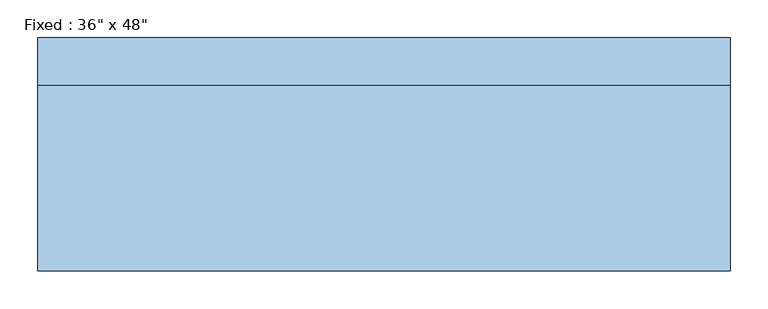
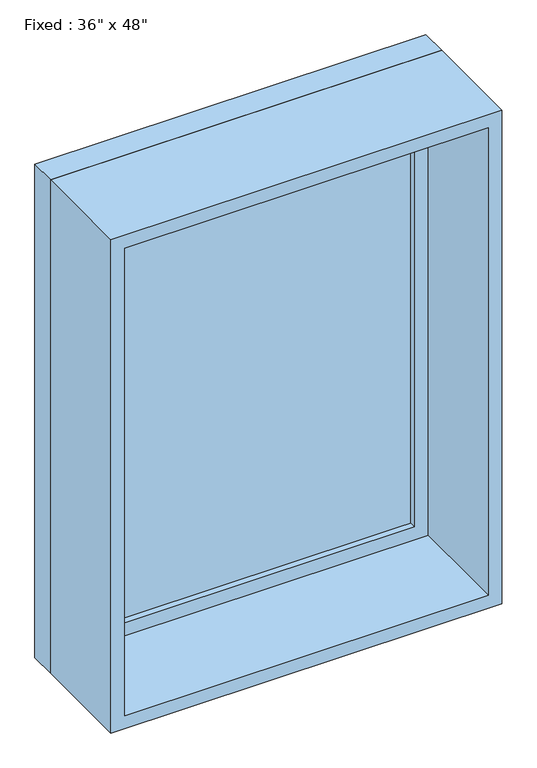
"""IFC4 building model written with IfcOpenShell, lengths in millimetres: window geometry."""

import ifcopenshell
import ifcopenshell.guid

model = None  # the IFC model being written
_history = None  # IfcOwnerHistory: only IFC2X3 demands one
_inside = {}  # id of a spatial element -> (the spatial element, [elements in it])
_under = {}  # id of a project, library or spatial element -> (it, [spatial elements below it])
_declared = {}  # id of a project -> (the project, [libraries it declares])
_typed = {}  # id of a type object -> (the type object, [elements of that type])
_made_of = {}  # id of a material, layer set ... -> (it, [elements and type objects made of it])


def new_model(schema):
    """Start an empty IFC model of exactly this schema.

    Asked for "IFC4X3", IfcOpenShell would pick the latest addendum, in which some entities
    have other attributes; the version numbers below select the first issue.
    IFC2X3 requires an IfcOwnerHistory on every rooted entity: one is made here for all.
    """
    global model, _history
    if schema == "IFC4X3":
        model = ifcopenshell.file(schema_version=(4, 3, 0, 0))
    else:
        model = ifcopenshell.file(schema=schema)
    _inside.clear()
    _under.clear()
    _declared.clear()
    _typed.clear()
    _made_of.clear()
    _history = None
    if model.schema == "IFC2X3":
        org = make("IfcOrganization", Name="unknown")
        user = make(
            "IfcPersonAndOrganization",
            ThePerson=make("IfcPerson", FamilyName="unknown"),
            TheOrganization=org,
        )
        app = make(
            "IfcApplication",
            ApplicationDeveloper=org,
            Version="unknown",
            ApplicationFullName="unknown",
            ApplicationIdentifier="unknown",
        )
        _history = make(
            "IfcOwnerHistory",
            OwningUser=user,
            OwningApplication=app,
            ChangeAction="ADDED",
            CreationDate=0,
        )
    return model


def make(cls, **values):
    """One entity of the class cls with the attributes given. An attribute that is None is left unset."""
    return model.create_entity(
        cls, **{name: value for name, value in values.items() if value is not None}
    )


def rooted(cls, **values):
    """An entity with a GlobalId (a new one), such as an element, a storey or a relation."""
    return make(cls, GlobalId=ifcopenshell.guid.new(), OwnerHistory=_history, **values)


def si_unit(unit_type, name, prefix=None):
    """IfcSIUnit, for example si_unit("LENGTHUNIT", "METRE", prefix="MILLI")."""
    return make("IfcSIUnit", UnitType=unit_type, Prefix=prefix, Name=name)


def assignment(units):
    """IfcUnitAssignment: the units of a project."""
    return None if units is None else make("IfcUnitAssignment", Units=units)


def point(xyz):
    """IfcCartesianPoint."""
    return None if xyz is None else make("IfcCartesianPoint", Coordinates=xyz)


def direction(xyz):
    """IfcDirection."""
    return None if xyz is None else make("IfcDirection", DirectionRatios=xyz)


def frame(location, z_axis=None, x_axis=None):
    """IfcAxis2Placement3D, a coordinate frame: its origin and axes. An axis left out is left unset."""
    return make(
        "IfcAxis2Placement3D",
        Location=point(location),
        Axis=direction(z_axis),
        RefDirection=direction(x_axis),
    )


def origin():
    """The frame at (0, 0, 0) with its axes left unset."""
    return frame((0.0, 0.0, 0.0))


def place(relative_to, where):
    """IfcLocalPlacement: puts the frame where relative to a parent placement (None: the world)."""
    return make(
        "IfcLocalPlacement", PlacementRelTo=relative_to, RelativePlacement=where
    )


def context(
    kind, dimensions, precision=None, world=None, true_north=None, identifier=None
):
    """IfcGeometricRepresentationContext, for example the 3D "Model" context."""
    return make(
        "IfcGeometricRepresentationContext",
        ContextIdentifier=identifier,
        ContextType=kind,
        CoordinateSpaceDimension=dimensions,
        Precision=precision,
        WorldCoordinateSystem=world,
        TrueNorth=true_north,
    )


def project(units=None, contexts=None):
    """IfcProject with its units and contexts."""
    return rooted(
        "IfcProject",
        Name="project",
        RepresentationContexts=contexts,
        UnitsInContext=assignment(units),
    )


def spatial(cls, under=None, at=None, **own):
    """A site, building, storey or space (cls), placed at a placement, below another one or the project."""
    s = rooted(cls, ObjectPlacement=at, **own)
    if under is not None:
        _under.setdefault(under.id(), (under, []))[1].append(s)
    return s


def polyline(points):
    """IfcPolyline through the points."""
    return make("IfcPolyline", Points=[point(p) for p in points])


def outline(outer, holes=None, kind="AREA"):
    """IfcArbitraryClosedProfileDef: a profile drawn as a closed curve; with holes, ...WithVoids."""
    if holes is None:
        return make("IfcArbitraryClosedProfileDef", ProfileType=kind, OuterCurve=outer)
    return make(
        "IfcArbitraryProfileDefWithVoids",
        ProfileType=kind,
        OuterCurve=outer,
        InnerCurves=holes,
    )


def extrude(swept, where, along, depth):
    """IfcExtrudedAreaSolid: the profile swept, set in the frame where, extruded along a direction by depth."""
    return make(
        "IfcExtrudedAreaSolid",
        SweptArea=swept,
        Position=where,
        ExtrudedDirection=direction(along),
        Depth=depth,
    )


def shape(context_of_items, identifier, shape_type, items):
    """IfcShapeRepresentation: the items that make up one representation, for example the "Body"."""
    return make(
        "IfcShapeRepresentation",
        ContextOfItems=context_of_items,
        RepresentationIdentifier=identifier,
        RepresentationType=shape_type,
        Items=items,
    )


def source(mapping_origin, context_of_items, identifier, shape_type, items):
    """IfcRepresentationMap: a shape defined once, which mapped items show again and again."""
    return make(
        "IfcRepresentationMap",
        MappingOrigin=mapping_origin,
        MappedRepresentation=shape(context_of_items, identifier, shape_type, items),
    )


def transform(
    local_origin,
    x_axis=None,
    y_axis=None,
    z_axis=None,
    scale=None,
    scale2=None,
    scale3=None,
    uniform=True,
):
    """IfcCartesianTransformationOperator3D, or its non-uniform kind. x_axis, y_axis, z_axis: its Axis1, 2, 3."""
    if uniform:
        return make(
            "IfcCartesianTransformationOperator3D",
            Axis1=direction(x_axis),
            Axis2=direction(y_axis),
            LocalOrigin=point(local_origin),
            Scale=scale,
            Axis3=direction(z_axis),
        )
    return make(
        "IfcCartesianTransformationOperator3DnonUniform",
        Axis1=direction(x_axis),
        Axis2=direction(y_axis),
        LocalOrigin=point(local_origin),
        Scale=scale,
        Axis3=direction(z_axis),
        Scale2=scale2,
        Scale3=scale3,
    )


def mapped(mapping_source, mapping_target):
    """IfcMappedItem: shows the shape of a source again, moved by a transform."""
    return make(
        "IfcMappedItem", MappingSource=mapping_source, MappingTarget=mapping_target
    )


def made_of(thing, what):
    """Note that an element or type object is made of a material, layer set ...; save() writes the relation."""
    if what is not None:
        _made_of.setdefault(what.id(), (what, []))[1].append(thing)
    return thing


def element(
    cls,
    number,
    at=None,
    inside=None,
    cuts=None,
    type_object=None,
    material=None,
    context=None,
    identifier="Body",
    shape_type=None,
    held_by="IfcProductDefinitionShape",
    body=None,
    shapes=None,
    **own,
):
    """One element of the class cls, such as IfcWall. Its Tag is "e" and its number.

    at: its placement. inside: the storey or other place that contains it. cuts: it is an
    opening in that element (IfcRelVoidsElement). A single representation is given by context,
    identifier, shape_type and body (its items); several are given by shapes. held_by: the class
    of the entity that holds the representations. save() writes the other relations.
    """
    e = rooted(cls, Tag="e%d" % number, ObjectPlacement=at, **own)
    if body is not None:
        shapes = [shape(context, identifier, shape_type, body)]
    if shapes is not None:
        e.Representation = make(held_by, Representations=shapes)
    if inside is not None:
        _inside.setdefault(inside.id(), (inside, []))[1].append(e)
    if cuts is not None:
        rooted(
            "IfcRelVoidsElement", RelatingBuildingElement=cuts, RelatedOpeningElement=e
        )
    if type_object is not None:
        _typed.setdefault(type_object.id(), (type_object, []))[1].append(e)
    return made_of(e, material)


def aggregate(whole, parts):
    """IfcRelAggregates: a whole, such as a stair, and the parts it consists of."""
    return rooted("IfcRelAggregates", RelatingObject=whole, RelatedObjects=parts)


def save(model, path):
    """Write the relations noted so far, then the file.

    IfcRelAggregates (storeys below a building ...), IfcRelContainedInSpatialStructure (elements
    in a storey), IfcRelDefinesByType, IfcRelAssociatesMaterial and IfcRelDeclares: one each for
    every whole, place, type object, material and project.
    """
    for whole, parts in _under.values():
        aggregate(whole, parts)
    for where, things in _inside.values():
        rooted(
            "IfcRelContainedInSpatialStructure",
            RelatedElements=things,
            RelatingStructure=where,
        )
    for kind, things in _typed.values():
        rooted("IfcRelDefinesByType", RelatedObjects=things, RelatingType=kind)
    for what, things in _made_of.values():
        rooted("IfcRelAssociatesMaterial", RelatedObjects=things, RelatingMaterial=what)
    for by, libraries in _declared.values():
        rooted("IfcRelDeclares", RelatingContext=by, RelatedDefinitions=libraries)
    model.write(path)


def window_dfee3f32(model_context):
    return source(origin(), model_context, "Body", "SweptSolid", [
        extrude(outline(polyline([(355.6, 106.3625), (-431.8, 106.3625), (-431.8, 119.0625), (355.6, 119.0625), (355.6, 106.3625)])), frame((0.0, 0.0, 977.9), z_axis=(0.0, 0.0, 1.0), x_axis=(1.0, 0.0, 0.0)), (0.0, 0.0, 1.0), 1092.2),
        extrude(outline(polyline([(2114.55, -476.25), (933.45, -476.25), (933.45, 400.05), (2114.55, 400.05), (2114.55, -476.25)]), holes=[polyline([(2070.1, -431.8), (2070.1, 355.6), (977.9, 355.6), (977.9, -431.8), (2070.1, -431.8)])]), frame((0.0, 90.4875, 0.0), z_axis=(0.0, 1.0, 0.0), x_axis=(0.0, 0.0, 1.0)), (0.0, 0.0, 1.0), 44.45),
        extrude(outline(polyline([(2133.6, -495.3), (914.4, -495.3), (914.4, 419.1), (2133.6, 419.1), (2133.6, -495.3)]), holes=[polyline([(2101.85, -463.55), (2101.85, 387.35), (946.15, 387.35), (946.15, -463.55), (2101.85, -463.55)])]), frame((0.0, -153.9875, 0.0), z_axis=(0.0, 1.0, 0.0), x_axis=(0.0, 0.0, 1.0)), (0.0, 0.0, 1.0), 244.475),
        extrude(outline(polyline([(2133.6, 419.1), (2133.6, -495.3), (914.4, -495.3), (914.4, 419.1), (2133.6, 419.1)]), holes=[polyline([(2114.55, 400.05), (933.45, 400.05), (933.45, -476.25), (2114.55, -476.25), (2114.55, 400.05)])]), frame((0.0, 90.4875, 0.0), z_axis=(0.0, 1.0, 0.0), x_axis=(0.0, 0.0, 1.0)), (0.0, 0.0, 1.0), 63.5),
    ])


if __name__ == "__main__":
    model = new_model("IFC4")
    model_context = context("Model", 3, world=origin())
    ifc_project = project(units=[si_unit("LENGTHUNIT", "METRE", prefix="MILLI")], contexts=[model_context])
    site = spatial("IfcSite", under=ifc_project)
    building = spatial("IfcBuilding", under=site)
    placement = place(None, origin())
    window_shape = window_dfee3f32(model_context)
    element("IfcWindow", 1, ObjectType="Fixed : 36\" x 48\"", at=placement, inside=building, context=model_context, shape_type="MappedRepresentation", body=[
        mapped(window_shape, transform((0.0, 0.0, 0.0), x_axis=(1.0, 0.0, 0.0), y_axis=(0.0, 1.0, 0.0), z_axis=(0.0, 0.0, 1.0))),
    ])
    save(model, "model.ifc")

# Revit data of these elements
# Type "Fixed : 36\" x 48\""
#   Type Mark = "1"
#   Assembly Code = "B2020100"
#   Height = 4' - 0"
#   Default Sill Height = 3' - 0"
#   Width = 3' - 0"
#   Window Inset = 0' - 0 3/4"
#   Glass Pane Material = Glass
#   Sash Material = Sash
#   Wall Closure = (empty or 0)
# Element 1 (IfcWindow, "Fixed : 36\" x 48\"")
#   Materials on its faces: "Sash", "Glass"
# Materials
#   "Glass": class "Glass", colour RGB 0 128 192, transparency 0.75
#   "Sash": class "Wood", colour RGB 224 178 126, transparency 0
